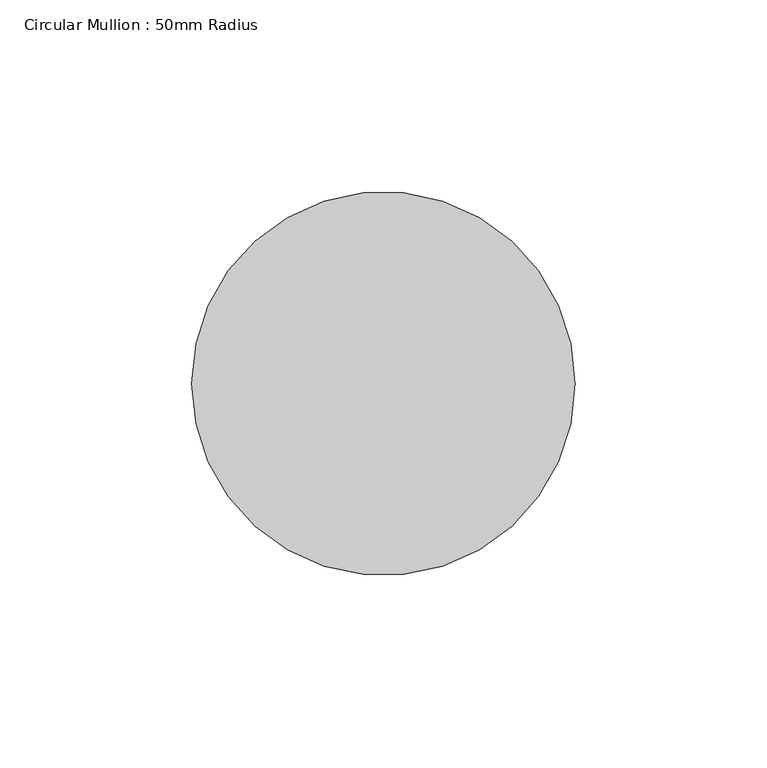
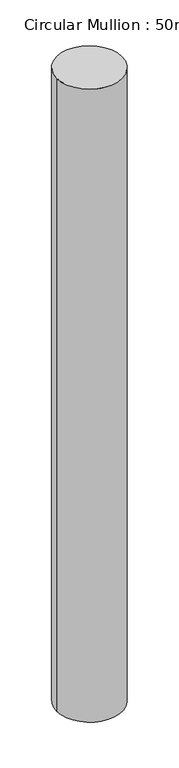
"""IFC4 building model written with IfcOpenShell, lengths in millimetres: member geometry, Circular Mullion : 50mm Radius."""

from ifc_helpers import new_model, si_unit, point, frame, origin, origin_2d, place, context, project, spatial, circle_curve, trimmed, segment, composite_curve, outline, extrude, source, transform, mapped, element, save


def circular_mullion_50mm_radius_965bf07d(model_context):
    return source(origin(), model_context, "Body", "SweptSolid", [
        extrude(outline(composite_curve([segment(trimmed(circle_curve(origin_2d(), 50.0), [point((50.0, 0.0))], [point((-50.0, 0.0))], False, "CARTESIAN"), True, "CONTINUOUS"), segment(trimmed(circle_curve(origin_2d(), 50.0), [point((-50.0, 0.0))], [point((50.0, 0.0))], False, "CARTESIAN"), True, "CONTINUOUS")], self_intersect=False)), frame((0.0, 0.0, -1020.4822402), z_axis=(0.0, 0.0, 1.0), x_axis=(1.0, 0.0, 0.0)), (0.0, 0.0, 1.0), 1020.4822402),
    ])


if __name__ == "__main__":
    model = new_model("IFC4")
    model_context = context("Model", 3, world=origin())
    ifc_project = project(units=[si_unit("LENGTHUNIT", "METRE", prefix="MILLI")], contexts=[model_context])
    site = spatial("IfcSite", under=ifc_project)
    building = spatial("IfcBuilding", under=site)
    placement = place(None, origin())
    circular_mullion_50mm_radius_shape = circular_mullion_50mm_radius_965bf07d(model_context)
    element("IfcMember", 1, ObjectType="Circular Mullion : 50mm Radius", at=placement, inside=building, context=model_context, shape_type="MappedRepresentation", body=[
        mapped(circular_mullion_50mm_radius_shape, transform((0.0, 0.0, 0.0), x_axis=(1.0, 0.0, 0.0), y_axis=(0.0, 1.0, 0.0), z_axis=(0.0, 0.0, 1.0))),
    ])
    save(model, "model.ifc")

# Revit data of these elements
# Type "Circular Mullion : 50mm Radius"
#   built-in parameter 1007350 = 0.164042 (stored number, unit not read)
# Element 1 (IfcMember, "Circular Mullion : 50mm Radius")
#   Materials on its faces: "Aluminium"
# Materials
#   "Aluminium": class "Metal", colour RGB 247 247 247, transparency 0, Description = "Aluminium 6061", Cost = 0
